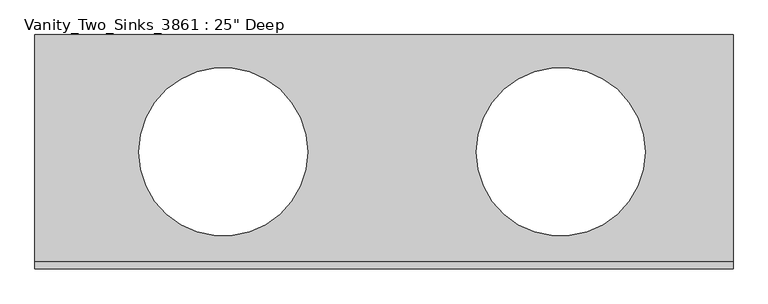
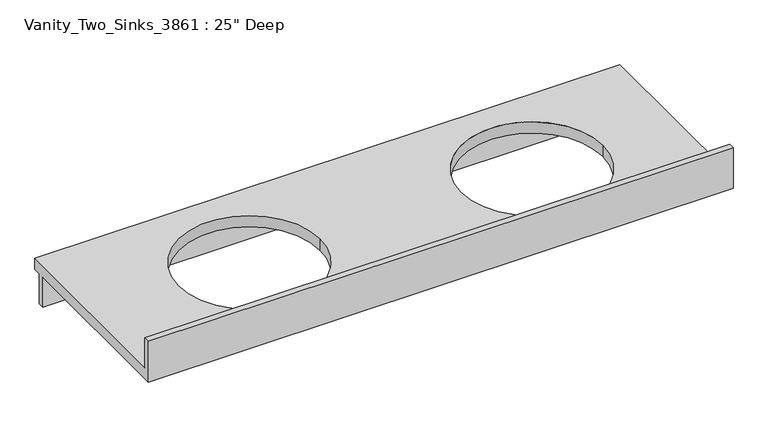
"""IFC4 building model written with IfcOpenShell, lengths in millimetres: furniture geometry."""

import ifcopenshell
import ifcopenshell.guid

model = None  # the IFC model being written
_history = None  # IfcOwnerHistory: only IFC2X3 demands one
_inside = {}  # id of a spatial element -> (the spatial element, [elements in it])
_under = {}  # id of a project, library or spatial element -> (it, [spatial elements below it])
_declared = {}  # id of a project -> (the project, [libraries it declares])
_typed = {}  # id of a type object -> (the type object, [elements of that type])
_made_of = {}  # id of a material, layer set ... -> (it, [elements and type objects made of it])


def new_model(schema):
    """Start an empty IFC model of exactly this schema.

    Asked for "IFC4X3", IfcOpenShell would pick the latest addendum, in which some entities
    have other attributes; the version numbers below select the first issue.
    IFC2X3 requires an IfcOwnerHistory on every rooted entity: one is made here for all.
    """
    global model, _history
    if schema == "IFC4X3":
        model = ifcopenshell.file(schema_version=(4, 3, 0, 0))
    else:
        model = ifcopenshell.file(schema=schema)
    _inside.clear()
    _under.clear()
    _declared.clear()
    _typed.clear()
    _made_of.clear()
    _history = None
    if model.schema == "IFC2X3":
        org = make("IfcOrganization", Name="unknown")
        user = make(
            "IfcPersonAndOrganization",
            ThePerson=make("IfcPerson", FamilyName="unknown"),
            TheOrganization=org,
        )
        app = make(
            "IfcApplication",
            ApplicationDeveloper=org,
            Version="unknown",
            ApplicationFullName="unknown",
            ApplicationIdentifier="unknown",
        )
        _history = make(
            "IfcOwnerHistory",
            OwningUser=user,
            OwningApplication=app,
            ChangeAction="ADDED",
            CreationDate=0,
        )
    return model


def make(cls, **values):
    """One entity of the class cls with the attributes given. An attribute that is None is left unset."""
    return model.create_entity(
        cls, **{name: value for name, value in values.items() if value is not None}
    )


def rooted(cls, **values):
    """An entity with a GlobalId (a new one), such as an element, a storey or a relation."""
    return make(cls, GlobalId=ifcopenshell.guid.new(), OwnerHistory=_history, **values)


def si_unit(unit_type, name, prefix=None):
    """IfcSIUnit, for example si_unit("LENGTHUNIT", "METRE", prefix="MILLI")."""
    return make("IfcSIUnit", UnitType=unit_type, Prefix=prefix, Name=name)


def assignment(units):
    """IfcUnitAssignment: the units of a project."""
    return None if units is None else make("IfcUnitAssignment", Units=units)


def point(xyz):
    """IfcCartesianPoint."""
    return None if xyz is None else make("IfcCartesianPoint", Coordinates=xyz)


def direction(xyz):
    """IfcDirection."""
    return None if xyz is None else make("IfcDirection", DirectionRatios=xyz)


def frame(location, z_axis=None, x_axis=None):
    """IfcAxis2Placement3D, a coordinate frame: its origin and axes. An axis left out is left unset."""
    return make(
        "IfcAxis2Placement3D",
        Location=point(location),
        Axis=direction(z_axis),
        RefDirection=direction(x_axis),
    )


def origin():
    """The frame at (0, 0, 0) with its axes left unset."""
    return frame((0.0, 0.0, 0.0))


def place(relative_to, where):
    """IfcLocalPlacement: puts the frame where relative to a parent placement (None: the world)."""
    return make(
        "IfcLocalPlacement", PlacementRelTo=relative_to, RelativePlacement=where
    )


def context(
    kind, dimensions, precision=None, world=None, true_north=None, identifier=None
):
    """IfcGeometricRepresentationContext, for example the 3D "Model" context."""
    return make(
        "IfcGeometricRepresentationContext",
        ContextIdentifier=identifier,
        ContextType=kind,
        CoordinateSpaceDimension=dimensions,
        Precision=precision,
        WorldCoordinateSystem=world,
        TrueNorth=true_north,
    )


def project(units=None, contexts=None):
    """IfcProject with its units and contexts."""
    return rooted(
        "IfcProject",
        Name="project",
        RepresentationContexts=contexts,
        UnitsInContext=assignment(units),
    )


def spatial(cls, under=None, at=None, **own):
    """A site, building, storey or space (cls), placed at a placement, below another one or the project."""
    s = rooted(cls, ObjectPlacement=at, **own)
    if under is not None:
        _under.setdefault(under.id(), (under, []))[1].append(s)
    return s


def polyline(points):
    """IfcPolyline through the points."""
    return make("IfcPolyline", Points=[point(p) for p in points])


def circle_curve(where, radius):
    """IfcCircle in the frame where."""
    return make("IfcCircle", Position=where, Radius=radius)


def shape(context_of_items, identifier, shape_type, items):
    """IfcShapeRepresentation: the items that make up one representation, for example the "Body"."""
    return make(
        "IfcShapeRepresentation",
        ContextOfItems=context_of_items,
        RepresentationIdentifier=identifier,
        RepresentationType=shape_type,
        Items=items,
    )


def source(mapping_origin, context_of_items, identifier, shape_type, items):
    """IfcRepresentationMap: a shape defined once, which mapped items show again and again."""
    return make(
        "IfcRepresentationMap",
        MappingOrigin=mapping_origin,
        MappedRepresentation=shape(context_of_items, identifier, shape_type, items),
    )


def transform(
    local_origin,
    x_axis=None,
    y_axis=None,
    z_axis=None,
    scale=None,
    scale2=None,
    scale3=None,
    uniform=True,
):
    """IfcCartesianTransformationOperator3D, or its non-uniform kind. x_axis, y_axis, z_axis: its Axis1, 2, 3."""
    if uniform:
        return make(
            "IfcCartesianTransformationOperator3D",
            Axis1=direction(x_axis),
            Axis2=direction(y_axis),
            LocalOrigin=point(local_origin),
            Scale=scale,
            Axis3=direction(z_axis),
        )
    return make(
        "IfcCartesianTransformationOperator3DnonUniform",
        Axis1=direction(x_axis),
        Axis2=direction(y_axis),
        LocalOrigin=point(local_origin),
        Scale=scale,
        Axis3=direction(z_axis),
        Scale2=scale2,
        Scale3=scale3,
    )


def mapped(mapping_source, mapping_target):
    """IfcMappedItem: shows the shape of a source again, moved by a transform."""
    return make(
        "IfcMappedItem", MappingSource=mapping_source, MappingTarget=mapping_target
    )


def made_of(thing, what):
    """Note that an element or type object is made of a material, layer set ...; save() writes the relation."""
    if what is not None:
        _made_of.setdefault(what.id(), (what, []))[1].append(thing)
    return thing


def element(
    cls,
    number,
    at=None,
    inside=None,
    cuts=None,
    type_object=None,
    material=None,
    context=None,
    identifier="Body",
    shape_type=None,
    held_by="IfcProductDefinitionShape",
    body=None,
    shapes=None,
    **own,
):
    """One element of the class cls, such as IfcWall. Its Tag is "e" and its number.

    at: its placement. inside: the storey or other place that contains it. cuts: it is an
    opening in that element (IfcRelVoidsElement). A single representation is given by context,
    identifier, shape_type and body (its items); several are given by shapes. held_by: the class
    of the entity that holds the representations. save() writes the other relations.
    """
    e = rooted(cls, Tag="e%d" % number, ObjectPlacement=at, **own)
    if body is not None:
        shapes = [shape(context, identifier, shape_type, body)]
    if shapes is not None:
        e.Representation = make(held_by, Representations=shapes)
    if inside is not None:
        _inside.setdefault(inside.id(), (inside, []))[1].append(e)
    if cuts is not None:
        rooted(
            "IfcRelVoidsElement", RelatingBuildingElement=cuts, RelatedOpeningElement=e
        )
    if type_object is not None:
        _typed.setdefault(type_object.id(), (type_object, []))[1].append(e)
    return made_of(e, material)


def aggregate(whole, parts):
    """IfcRelAggregates: a whole, such as a stair, and the parts it consists of."""
    return rooted("IfcRelAggregates", RelatingObject=whole, RelatedObjects=parts)


def save(model, path):
    """Write the relations noted so far, then the file.

    IfcRelAggregates (storeys below a building ...), IfcRelContainedInSpatialStructure (elements
    in a storey), IfcRelDefinesByType, IfcRelAssociatesMaterial and IfcRelDeclares: one each for
    every whole, place, type object, material and project.
    """
    for whole, parts in _under.values():
        aggregate(whole, parts)
    for where, things in _inside.values():
        rooted(
            "IfcRelContainedInSpatialStructure",
            RelatedElements=things,
            RelatingStructure=where,
        )
    for kind, things in _typed.values():
        rooted("IfcRelDefinesByType", RelatedObjects=things, RelatingType=kind)
    for what, things in _made_of.values():
        rooted("IfcRelAssociatesMaterial", RelatedObjects=things, RelatingMaterial=what)
    for by, libraries in _declared.values():
        rooted("IfcRelDeclares", RelatingContext=by, RelatedDefinitions=libraries)
    model.write(path)


def plane_surface(at):
    """IfcPlane: the flat surface through the origin of the frame at, square to its z axis."""
    return make("IfcPlane", Position=at)


def revolved_surface(curve, axis_point, axis_direction):
    """IfcSurfaceOfRevolution: the curve turned about the line through axis_point along axis_direction."""
    return make(
        "IfcSurfaceOfRevolution",
        SweptCurve=make("IfcArbitraryOpenProfileDef", ProfileType="CURVE", Curve=curve),
        AxisPosition=make("IfcAxis1Placement", Location=point(axis_point), Axis=direction(axis_direction)),
    )


def advanced_brep(points, edges, surfaces, faces):
    """IfcAdvancedBrep: a solid bounded by faces that lie on surfaces and meet in shared edges.

    An edge is (start, end): straight between two places in points (the first is 0);
    or (start, end, curve); or (start, end, curve, False) where it runs against its curve.
    A face is (place in surfaces, loops), or (place, loops, False) where it looks against
    its surface's normal. A loop lists edges by number (the first is 1), with a minus sign
    where the edge is run from its end to its start. The first loop is the outer one.
    """
    corners = [point(p) for p in points]
    vertices = [make("IfcVertexPoint", VertexGeometry=c) for c in corners]
    made = []
    for start, end, *more in edges:
        made.append(
            make(
                "IfcEdgeCurve",
                EdgeStart=vertices[start],
                EdgeEnd=vertices[end],
                EdgeGeometry=more[0] if more else make("IfcPolyline", Points=[corners[start], corners[end]]),
                SameSense=more[1] if len(more) > 1 else True,
            )
        )
    hull = []
    for where, loops, *sense in faces:
        bounds = []
        for j, loop in enumerate(loops):
            ring = [make("IfcOrientedEdge", EdgeElement=made[abs(k) - 1], Orientation=k > 0) for k in loop]
            bounds.append(
                make(
                    "IfcFaceOuterBound" if j == 0 else "IfcFaceBound",
                    Bound=make("IfcEdgeLoop", EdgeList=ring),
                    Orientation=True,
                )
            )
        hull.append(make("IfcAdvancedFace", Bounds=bounds, FaceSurface=surfaces[where], SameSense=sense[0] if sense else True))
    return make("IfcAdvancedBrep", Outer=make("IfcClosedShell", CfsFaces=hull))


def furniture_6b9eb554(model_context):
    return source(origin(), model_context, "Body", "AdvancedBrep", [
        advanced_brep(
        [(-1327.4622951, 635.0, 863.6), (-1327.4622951, 19.05, 863.6), (564.3712969, 19.05, 863.6), (564.3712969, 635.0, 863.6), (325.7362884, 317.5, 863.6), (-131.4637116, 317.5, 863.6), (-588.6637116, 317.5, 863.6), (-1045.8637116, 317.5, 863.6), (564.3712969, 635.0, 825.5), (564.3712969, 609.6, 825.5), (-1327.4622951, 609.6, 825.5), (-1327.4622951, 635.0, 825.5), (-1327.4622951, 0.0, 825.5), (-1327.4622951, 590.55, 825.5), (564.3712969, 590.55, 825.5), (564.3712969, 0.0, 825.5), (-131.4637116, 317.5, 825.5), (325.7362884, 317.5, 825.5), (-1045.8637116, 317.5, 825.5), (-588.6637116, 317.5, 825.5), (564.3712969, 0.0, 965.2), (-1327.4622951, 0.0, 965.2), (-1327.4622951, 609.6, 723.9), (-1327.4622951, 590.55, 723.9), (-1327.4622951, 19.05, 965.2), (564.3712969, 19.05, 965.2), (564.3712969, 590.55, 723.9), (564.3712969, 609.6, 723.9)],
        [
            (0, 1),
            (1, 2),
            (2, 3),
            (3, 0),
            (4, 5, circle_curve(frame((97.1362884, 317.5, 863.6), z_axis=(0.0, 0.0, -1.0), x_axis=(1.0, 0.0, 0.0)), 228.6)),
            (5, 4, circle_curve(frame((97.1362884, 317.5, 863.6), z_axis=(0.0, 0.0, -1.0), x_axis=(1.0, 0.0, 0.0)), 228.6)),
            (6, 7, circle_curve(frame((-817.2637116, 317.5, 863.6), z_axis=(0.0, 0.0, -1.0), x_axis=(1.0, 0.0, 0.0)), 228.6)),
            (7, 6, circle_curve(frame((-817.2637116, 317.5, 863.6), z_axis=(0.0, 0.0, -1.0), x_axis=(1.0, 0.0, 0.0)), 228.6)),
            (8, 9),
            (9, 10),
            (10, 11),
            (11, 8),
            (12, 13),
            (13, 14),
            (14, 15),
            (15, 12),
            (16, 17, circle_curve(frame((97.1362884, 317.5, 825.5), z_axis=(0.0, 0.0, 1.0), x_axis=(1.0, 0.0, 0.0)), 228.6)),
            (17, 16, circle_curve(frame((97.1362884, 317.5, 825.5), z_axis=(0.0, 0.0, 1.0), x_axis=(1.0, 0.0, 0.0)), 228.6)),
            (18, 19, circle_curve(frame((-817.2637116, 317.5, 825.5), z_axis=(0.0, 0.0, 1.0), x_axis=(1.0, 0.0, 0.0)), 228.6)),
            (19, 18, circle_curve(frame((-817.2637116, 317.5, 825.5), z_axis=(0.0, 0.0, 1.0), x_axis=(1.0, 0.0, 0.0)), 228.6)),
            (15, 20),
            (20, 21),
            (21, 12),
            (10, 22),
            (22, 23),
            (23, 13),
            (21, 24),
            (24, 1),
            (0, 11),
            (3, 8),
            (2, 25),
            (25, 20),
            (14, 26),
            (26, 27),
            (27, 9),
            (5, 16),
            (17, 4),
            (25, 24),
            (7, 18),
            (19, 6),
            (26, 23),
            (22, 27),
        ],
        [
            plane_surface(frame((-1327.4622951, 0.0, 863.6), z_axis=(0.0, 0.0, 1.0), x_axis=(-1.0, 0.0, 0.0))),
            plane_surface(frame((-1327.4622951, 0.0, 825.5), z_axis=(0.0, 0.0, -1.0), x_axis=(1.0, 0.0, 0.0))),
            plane_surface(frame((564.3712969, 0.0, 863.6), z_axis=(0.0, -1.0, 0.0), x_axis=(0.0, 0.0, -1.0))),
            plane_surface(frame((-1327.4622951, 0.0, 863.6), z_axis=(-1.0, 0.0, 0.0), x_axis=(0.0, 0.0, -1.0))),
            plane_surface(frame((-1327.4622951, 635.0, 863.6), z_axis=(0.0, 1.0, 0.0), x_axis=(0.0, 0.0, -1.0))),
            plane_surface(frame((564.3712969, 635.0, 863.6), z_axis=(1.0, 0.0, 0.0), x_axis=(0.0, 0.0, -1.0))),
            revolved_surface(polyline([(325.7362884, 317.5, 863.6), (325.7362884, 317.5, 825.5)]), (97.1362884, 317.5, 825.5), (0.0, 0.0, 1.0)),
            plane_surface(frame((-1327.4622951, 0.0, 965.2), z_axis=(0.0, 0.0, 1.0), x_axis=(0.0, 1.0, 0.0))),
            plane_surface(frame((-1327.4622951, 19.05, 965.2), z_axis=(0.0, 1.0, 0.0), x_axis=(0.0, 0.0, -1.0))),
            revolved_surface(polyline([(-588.6637115999999, 317.5, 863.6), (-588.6637115999999, 317.5, 825.5)]), (-817.2637116, 317.5, 825.5), (0.0, 0.0, 1.0)),
            plane_surface(frame((-1327.4622951, 590.55, 723.9), z_axis=(0.0, 0.0, -1.0), x_axis=(1.0, 0.0, 0.0))),
            plane_surface(frame((564.3712969, 590.55, 825.5), z_axis=(0.0, -1.0, 0.0), x_axis=(0.0, 0.0, -1.0))),
            plane_surface(frame((-1327.4622951, 609.6, 825.5), z_axis=(0.0, 1.0, 0.0), x_axis=(0.0, 0.0, -1.0))),
        ],
        [
            (0, [[1, 2, 3, 4], [5, 6], [7, 8]]),
            (1, [[9, 10, 11, 12]]),
            (1, [[13, 14, 15, 16], [17, 18], [19, 20]]),
            (2, [[21, 22, 23, -16]]),
            (3, [[-11, 24, 25, 26, -13, -23, 27, 28, -1, 29]]),
            (4, [[30, -12, -29, -4]]),
            (5, [[-3, 31, 32, -21, -15, 33, 34, 35, -9, -30]]),
            (6, [[-6, 36, -18, 37]]),
            (6, [[-17, -36, -5, -37]]),
            (7, [[-22, -32, 38, -27]]),
            (8, [[-31, -2, -28, -38]]),
            (9, [[-8, 39, -20, 40]]),
            (9, [[-19, -39, -7, -40]]),
            (10, [[41, -25, 42, -34]]),
            (11, [[-33, -14, -26, -41]]),
            (12, [[-24, -10, -35, -42]]),
        ],
    ),
    ])


if __name__ == "__main__":
    model = new_model("IFC4")
    model_context = context("Model", 3, world=origin())
    ifc_project = project(units=[si_unit("LENGTHUNIT", "METRE", prefix="MILLI")], contexts=[model_context])
    site = spatial("IfcSite", under=ifc_project)
    building = spatial("IfcBuilding", under=site)
    placement = place(None, origin())
    furniture_shape = furniture_6b9eb554(model_context)
    element("IfcFurniture", 1, ObjectType="Vanity_Two_Sinks_3861 : 25\" Deep", at=placement, inside=building, context=model_context, shape_type="MappedRepresentation", body=[
        mapped(furniture_shape, transform((0.0, 0.0, 0.0), x_axis=(1.0, 0.0, 0.0), y_axis=(0.0, 1.0, 0.0), z_axis=(0.0, 0.0, 1.0))),
    ])
    save(model, "model.ifc")

# Revit data of these elements
# Type "Vanity_Two_Sinks_3861 : 25\" Deep"
#   Assembly Code = "C1030400"
#   Sink Location Right [instance default] = 1' - 6"
#   Counter Thickness = 0' - 1 1/2"
#   Depth = 2' - 1"
#   Height = 2' - 10"
#   Length [instance default] = 6' - 0"
#   Sink Location Left [instance default] = 1' - 6"
#   Sink to Back Wall = 0' - 4"
#   Sink Opening Width [instance default] = 1' - 5"
#   Counter Top = Casework - Vanity Top
#   Width = 0
# Element 1 (IfcFurniture, "Vanity_Two_Sinks_3861 : 25\" Deep")
#   Sink Location Right = 1' - 6.39508"
#   Length = 6' - 2.48164"
#   Sink Location Left = 1' - 8.08656"
#   Materials on its faces: "Casework - Vanity Top"
# Materials
#   "Casework - Vanity Top": class "Unassigned", colour RGB 210 200 171, transparency 0, Comments = "Rendering appearance not upgraded "
